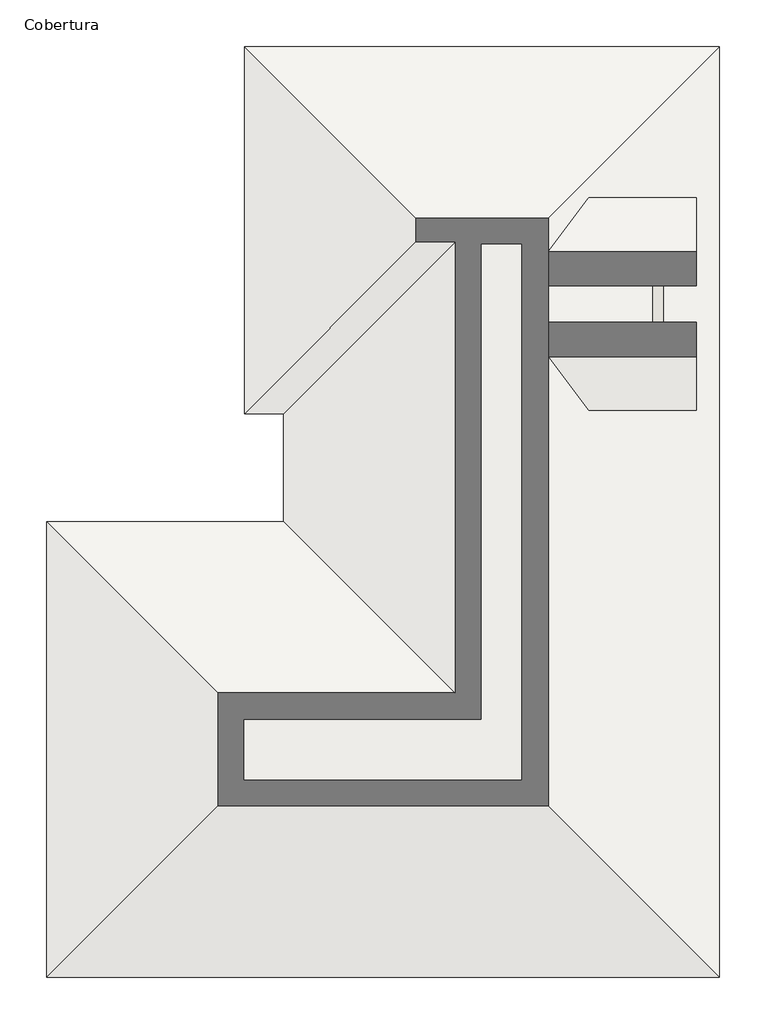
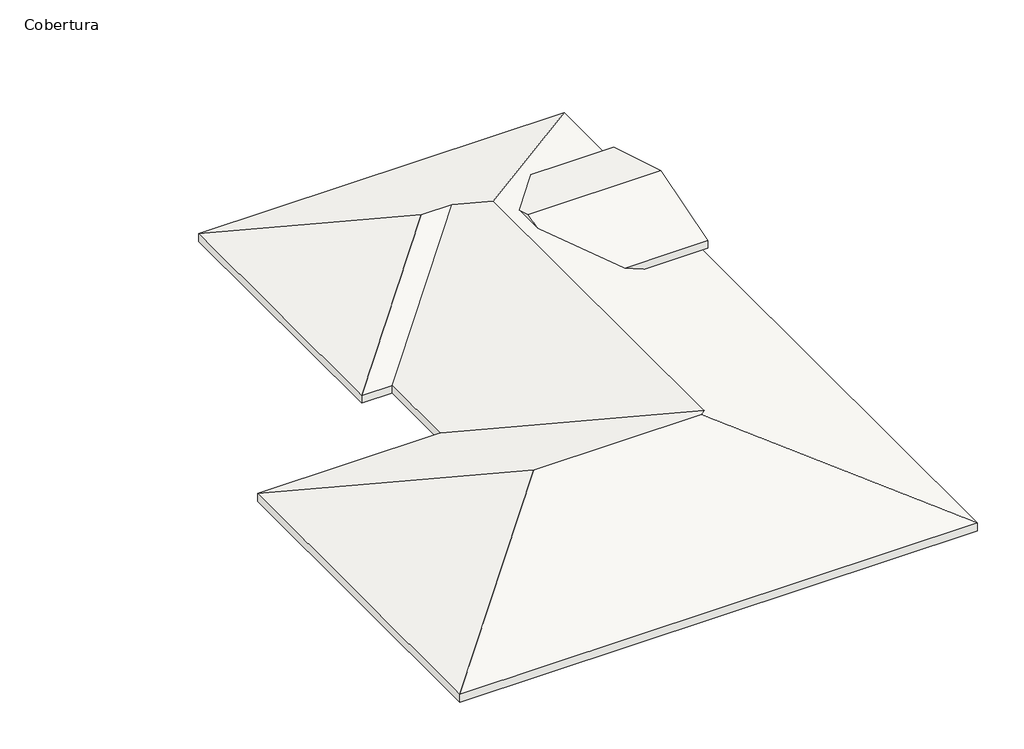
# One storey: 3 walls, 2 roofs, 1 slab.
"""IFC4 building model written with IfcOpenShell, lengths in millimetres."""

from ifc_helpers import new_model, si_unit, frame, origin, place, context, project, spatial, polyline, outline, extrude, faceted_brep, element, save

model = new_model("IFC4")

# Units and contexts
model_context = context("Model", 3, world=origin())
ifc_project = project(units=[si_unit("LENGTHUNIT", "METRE", prefix="MILLI")], contexts=[model_context])

# Site, building, storey
site = spatial("IfcSite", under=ifc_project)
building = spatial("IfcBuilding", under=site)
storey = spatial("IfcBuildingStorey", under=building, Name="Cobertura", Elevation=6400.0)

# Roofs
placement = place(None, origin())
element("IfcRoof", 1, ObjectType="Telhado 1", at=placement, inside=storey, context=model_context, shape_type="Brep", body=[
    faceted_brep([(-2702.5171244, 6323.9034535, 6400.0), (4505.125551, 6323.9034535, 6400.0), (1200.325551, 3019.1034535, 7721.92), (679.175551, 3540.2534535, 7513.46), (81.1328756, 3540.2534535, 7513.46), (-2702.5171244, 756.6034535, 6400.0), (-2104.474449, -883.7965465, 6400.0), (1200.325551, -4188.5965465, 7721.92), (1050.125551, -4338.7965465, 7782.0), (-2249.874449, -4338.7965465, 7782.0), (-5704.874449, -883.7965465, 6400.0), (-5704.874449, -7793.7965465, 6400.0), (4505.125551, -7793.7965465, 6400.0), (-2702.5171244, 6323.9034535, 6561.5549442), (81.1328756, 3540.2534535, 7675.0149442), (679.175551, 3540.2534535, 7675.0149442), (1200.325551, 3019.1034535, 7883.4749442), (4505.125551, 6323.9034535, 6561.5549442), (-2702.5171244, 756.6034535, 6561.5549442), (-2104.474449, -883.7965465, 6561.5549442), (-5704.874449, -883.7965465, 6561.5549442), (-2249.874449, -4338.7965465, 7943.5549442), (1050.125551, -4338.7965465, 7943.5549442), (1200.325551, -4188.5965465, 7883.4749442), (-5704.874449, -7793.7965465, 6561.5549442), (4505.125551, -7793.7965465, 6561.5549442), (-2104.474449, 756.6034535, 6400.0), (-2104.474449, 756.6034535, 6561.5549442)], [[[0, 1, 2, 3, 4]], [[0, 4, 5]], [[6, 7, 8, 9, 10]], [[11, 9, 8, 12]], [[10, 9, 11]], [[12, 8, 7, 2, 1]], [[13, 14, 15, 16, 17]], [[13, 18, 14]], [[19, 20, 21, 22, 23]], [[24, 25, 22, 21]], [[20, 24, 21]], [[25, 17, 16, 23, 22]], [[5, 18, 13, 0]], [[10, 20, 19, 6]], [[11, 24, 20, 10]], [[12, 25, 24, 11]], [[1, 17, 25, 12]], [[0, 13, 17, 1]], [[26, 5, 4, 3]], [[26, 3, 2, 7, 6]], [[18, 27, 15, 14]], [[27, 19, 23, 16, 15]], [[26, 27, 18, 5]], [[6, 19, 27, 26]]]),
])
element("IfcRoof", 2, ObjectType="Telhado 1", at=placement, inside=storey, context=model_context, shape_type="SweptSolid", body=[
    extrude(outline(polyline([(811.4833497, 7356.6045976), (2420.6833497, 7839.3645976), (4029.8833497, 7356.6045976), (4029.8833497, 7200.0), (2420.6833497, 7682.76), (811.4833497, 7200.0), (811.4833497, 7356.6045976)])), frame((1545.525551, 0.0, 0.0), z_axis=(1.0, 0.0, 0.0), x_axis=(0.0, 1.0, 0.0)), (0.0, 0.0, 1.0), 2609.2),
])

# Slab
element("IfcSlab", 3, ObjectType="Laje 10 cm", at=placement, inside=storey, context=model_context, shape_type="SweptSolid", body=[
    extrude(outline(polyline([(-1552.9171244, 5323.9034535), (3505.125551, 5323.9034535), (3505.125551, 428.5034535), (3505.125551, -805.4038456), (3505.125551, -6793.7965465), (-4704.874449, -6793.7965465), (-4704.874449, -1883.7965465), (-954.874449, -1883.7965465), (-954.874449, 1906.2034535), (-1552.9171244, 1906.2034535), (-1552.9171244, 5323.9034535)])), frame((0.0, 0.0, 6250.0), z_axis=(0.0, 0.0, 1.0), x_axis=(1.0, 0.0, 0.0)), (0.0, 0.0, 1.0), 150.0),
])

# Walls
element("IfcWall", 4, ObjectType="Parede Bloco 14 cm - Pintura / Pintura", at=placement, inside=storey, context=model_context, shape_type="Brep", body=[
    faceted_brep([(2045.525551, 3370.6833497, 6400.0), (3495.525551, 3370.6833497, 6400.0), (3495.525551, 3370.6833497, 6702.88), (3654.725551, 3370.6833497, 6702.88), (3654.725551, 3370.6833497, 7200.0), (3495.525551, 3370.6833497, 7200.0), (2045.525551, 3370.6833497, 7200.0), (2045.525551, 3529.8833497, 6400.0), (2045.525551, 3529.8833497, 7200.0), (3654.725551, 3529.8833497, 7200.0), (3654.725551, 3529.8833497, 6702.88), (3495.525551, 3529.8833497, 6702.88), (3495.525551, 3529.8833497, 6400.0)], [[[0, 1, 2, 3, 4, 5, 6]], [[7, 8, 9, 10, 11, 12]], [[1, 0, 7, 12]], [[6, 5, 4, 9, 8]], [[0, 6, 8, 7]], [[10, 3, 2, 11]], [[2, 1, 12, 11]], [[4, 3, 10, 9]]]),
])
element("IfcWall", 5, ObjectType="Parede Bloco 14 cm - Pintura / Pintura", at=placement, inside=storey, context=model_context, shape_type="Brep", body=[
    faceted_brep([(2055.125551, 1311.4833497, 6400.0), (3495.525551, 1311.4833497, 6400.0), (3495.525551, 1311.4833497, 6702.88), (3654.725551, 1311.4833497, 6702.88), (3654.725551, 1311.4833497, 7200.0), (2055.125551, 1311.4833497, 7200.0), (2055.125551, 1470.6833497, 6400.0), (2055.125551, 1470.6833497, 7200.0), (3495.525551, 1470.6833497, 7200.0), (3654.725551, 1470.6833497, 7200.0), (3654.725551, 1470.6833497, 6702.88), (3495.525551, 1470.6833497, 6702.88), (3495.525551, 1470.6833497, 6400.0)], [[[0, 1, 2, 3, 4, 5]], [[6, 7, 8, 9, 10, 11, 12]], [[1, 0, 6, 12]], [[5, 4, 9, 8, 7]], [[0, 5, 7, 6]], [[10, 3, 2, 11]], [[2, 1, 12, 11]], [[4, 3, 10, 9]]]),
])
element("IfcWall", 6, ObjectType="Parede Bloco 14 cm - Pintura / Pintura", at=placement, inside=storey, context=model_context, shape_type="Brep", body=[
    faceted_brep([(3495.525551, 3370.6833497, 6400.0), (3495.525551, 1470.6833497, 6400.0), (3495.525551, 1470.6833497, 7200.0), (3495.525551, 3370.6833497, 7200.0), (3654.725551, 3370.6833497, 6400.0), (3654.725551, 3370.6833497, 6702.88), (3654.725551, 3370.6833497, 7200.0), (3654.725551, 1470.6833497, 7200.0), (3654.725551, 1470.6833497, 6702.88), (3654.725551, 1470.6833497, 6400.0)], [[[0, 1, 2, 3]], [[4, 5, 6, 7, 8, 9]], [[1, 0, 4, 9]], [[3, 2, 7, 6]], [[0, 3, 6, 5, 4]], [[2, 1, 9, 8, 7]]]),
])

save(model, "model.ifc")

# Revit data of these elements
# Project information
#   Project Issue Date = "Data de emissão"
#   Project Status = "Status do projeto"
#   Client Name = "Proprietário"
#   Project Address = "Insira aqui o endereço"
#   Project Name = "Nome do projeto"
#   Project Number = "0001"
# Type "Telhado 1"
#   built-in parameter 1001600 = 0.492126 (stored number, unit not read)
#   Layers, outside or top first: 0.15 m "Telha cerâmica" (function 1)
# Type "Laje 10 cm"
#   Thickness = 0.15 m
#   Function = 0
#   Layers, outside or top first: 0.05 m "Cimentado Desempenado" (function 4); 0.10 m "Concreto" (function 1)
# Type "Parede Bloco 14 cm - Pintura / Pintura"
#   Width = 0.1592 m
#   Layers, outside or top first: 0.0016 m "Pintura Látex PVA" (function 4); 0.008 m "Gesso" (function 4); 0.14 m "Alvenaria - Bloco de Cerâmico" (function 1); 0.008 m "Gesso" (function 2); 0.0016 m "Pintura Látex PVA" (function 4)
# Element 1 (IfcRoof, "Telhado 1")
#   built-in parameter 1001705 = 26.0615 (stored number, unit not read)
#   built-in parameter 1001710 = 33615
#   Phase Created = Construção nova
#   Materials on its faces: "Telha cerâmica"
# Element 2 (IfcRoof, "Telhado 1")
#   built-in parameter 1001705 = 25.7197 (stored number, unit not read)
#   built-in parameter 1001701 = 2.62467 (stored number, unit not read)
#   built-in parameter 1001710 = 33615
#   Phase Created = Construção nova
#   Materials on its faces: "Telha cerâmica"
# Element 3 (IfcSlab, "Laje 10 cm")
#   built-in parameter 1001955 = 3.14159 (stored number, unit not read)
#   Height Offset From Level = 0.00 m
#   Phase Created = Construção nova
#   Materials on its faces: "Concreto", "Cimentado Desempenado"
# Elements 4, 5, 6 (IfcWall, "Parede Bloco 14 cm - Pintura / Pintura")
#   Top Offset = 0.00 m
#   Base Offset = 0.00 m
#   Unconnected Height = 0.80 m
#   wall height = 0.80 m
#   Phase Created = Construção nova
#   Base Constraint = Cobertura
#   Materials on its faces: "Material pré-definido de parede", "Pintura Látex PVA"
# Materials
#   "Telha cerâmica": class "Metal", colour RGB 166 82 82, transparency 0, Description = "Azulejo de telhado de barro", Cost = 0
#   "Cimentado Desempenado": class "Cimento", colour RGB 192 192 192, transparency 0, Cost = 0
#   "Concreto": class "Concreto", colour RGB 192 192 192, transparency 0, Cost = 0
#   "Pintura Látex PVA": class "Pintura", colour RGB 244 244 244, transparency 0, Cost = 0
#   "Gesso": class "Gesso", colour RGB 244 244 244, transparency 0, Cost = 0
#   "Alvenaria - Bloco de Cerâmico": class "Cerâmica", colour RGB 192 192 192, transparency 0, Cost = 0
#   "Material pré-definido de parede": class "Diversos", colour RGB 128 128 128, transparency 0
